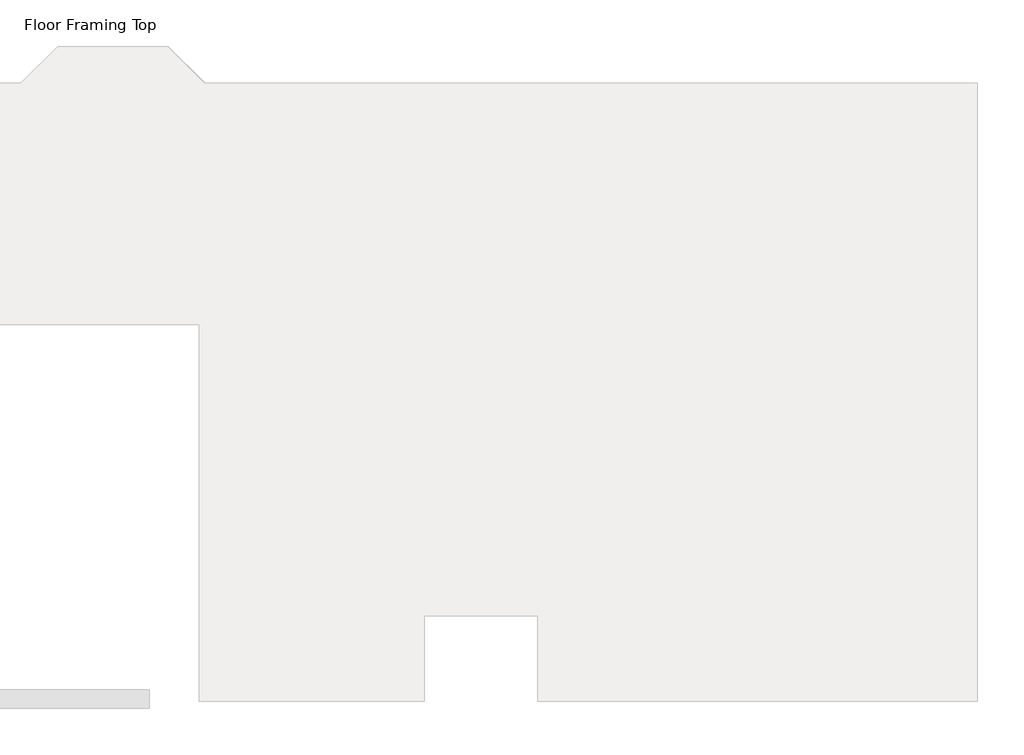
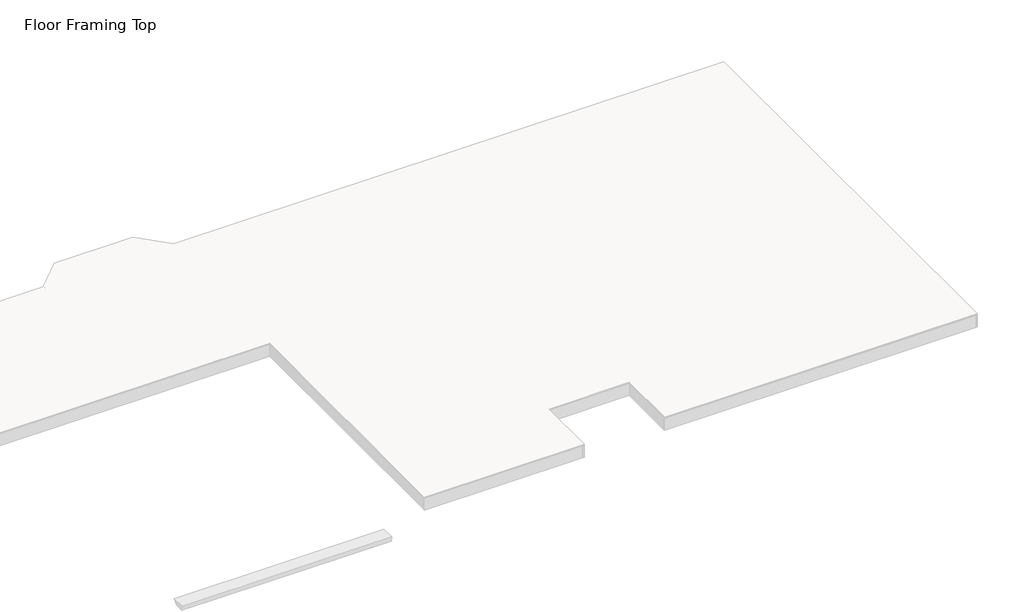
# One storey, part 2 of 4: 23 beams.
"""IFC4 building model written with IfcOpenShell, lengths in millimetres."""

import ifcopenshell
import ifcopenshell.guid

model = None  # the IFC model being written
_history = None  # IfcOwnerHistory: only IFC2X3 demands one
_inside = {}  # id of a spatial element -> (the spatial element, [elements in it])
_under = {}  # id of a project, library or spatial element -> (it, [spatial elements below it])
_declared = {}  # id of a project -> (the project, [libraries it declares])
_typed = {}  # id of a type object -> (the type object, [elements of that type])
_made_of = {}  # id of a material, layer set ... -> (it, [elements and type objects made of it])


def new_model(schema):
    """Start an empty IFC model of exactly this schema.

    Asked for "IFC4X3", IfcOpenShell would pick the latest addendum, in which some entities
    have other attributes; the version numbers below select the first issue.
    IFC2X3 requires an IfcOwnerHistory on every rooted entity: one is made here for all.
    """
    global model, _history
    if schema == "IFC4X3":
        model = ifcopenshell.file(schema_version=(4, 3, 0, 0))
    else:
        model = ifcopenshell.file(schema=schema)
    _inside.clear()
    _under.clear()
    _declared.clear()
    _typed.clear()
    _made_of.clear()
    _history = None
    if model.schema == "IFC2X3":
        org = make("IfcOrganization", Name="unknown")
        user = make(
            "IfcPersonAndOrganization",
            ThePerson=make("IfcPerson", FamilyName="unknown"),
            TheOrganization=org,
        )
        app = make(
            "IfcApplication",
            ApplicationDeveloper=org,
            Version="unknown",
            ApplicationFullName="unknown",
            ApplicationIdentifier="unknown",
        )
        _history = make(
            "IfcOwnerHistory",
            OwningUser=user,
            OwningApplication=app,
            ChangeAction="ADDED",
            CreationDate=0,
        )
    return model


def make(cls, **values):
    """One entity of the class cls with the attributes given. An attribute that is None is left unset."""
    return model.create_entity(
        cls, **{name: value for name, value in values.items() if value is not None}
    )


def rooted(cls, **values):
    """An entity with a GlobalId (a new one), such as an element, a storey or a relation."""
    return make(cls, GlobalId=ifcopenshell.guid.new(), OwnerHistory=_history, **values)


def si_unit(unit_type, name, prefix=None):
    """IfcSIUnit, for example si_unit("LENGTHUNIT", "METRE", prefix="MILLI")."""
    return make("IfcSIUnit", UnitType=unit_type, Prefix=prefix, Name=name)


def assignment(units):
    """IfcUnitAssignment: the units of a project."""
    return None if units is None else make("IfcUnitAssignment", Units=units)


def point(xyz):
    """IfcCartesianPoint."""
    return None if xyz is None else make("IfcCartesianPoint", Coordinates=xyz)


def direction(xyz):
    """IfcDirection."""
    return None if xyz is None else make("IfcDirection", DirectionRatios=xyz)


def frame(location, z_axis=None, x_axis=None):
    """IfcAxis2Placement3D, a coordinate frame: its origin and axes. An axis left out is left unset."""
    return make(
        "IfcAxis2Placement3D",
        Location=point(location),
        Axis=direction(z_axis),
        RefDirection=direction(x_axis),
    )


def origin():
    """The frame at (0, 0, 0) with its axes left unset."""
    return frame((0.0, 0.0, 0.0))


def place(relative_to, where):
    """IfcLocalPlacement: puts the frame where relative to a parent placement (None: the world)."""
    return make(
        "IfcLocalPlacement", PlacementRelTo=relative_to, RelativePlacement=where
    )


def context(
    kind, dimensions, precision=None, world=None, true_north=None, identifier=None
):
    """IfcGeometricRepresentationContext, for example the 3D "Model" context."""
    return make(
        "IfcGeometricRepresentationContext",
        ContextIdentifier=identifier,
        ContextType=kind,
        CoordinateSpaceDimension=dimensions,
        Precision=precision,
        WorldCoordinateSystem=world,
        TrueNorth=true_north,
    )


def project(units=None, contexts=None):
    """IfcProject with its units and contexts."""
    return rooted(
        "IfcProject",
        Name="project",
        RepresentationContexts=contexts,
        UnitsInContext=assignment(units),
    )


def spatial(cls, under=None, at=None, **own):
    """A site, building, storey or space (cls), placed at a placement, below another one or the project."""
    s = rooted(cls, ObjectPlacement=at, **own)
    if under is not None:
        _under.setdefault(under.id(), (under, []))[1].append(s)
    return s


def polyline(points):
    """IfcPolyline through the points."""
    return make("IfcPolyline", Points=[point(p) for p in points])


def outline(outer, holes=None, kind="AREA"):
    """IfcArbitraryClosedProfileDef: a profile drawn as a closed curve; with holes, ...WithVoids."""
    if holes is None:
        return make("IfcArbitraryClosedProfileDef", ProfileType=kind, OuterCurve=outer)
    return make(
        "IfcArbitraryProfileDefWithVoids",
        ProfileType=kind,
        OuterCurve=outer,
        InnerCurves=holes,
    )


def extrude(swept, where, along, depth):
    """IfcExtrudedAreaSolid: the profile swept, set in the frame where, extruded along a direction by depth."""
    return make(
        "IfcExtrudedAreaSolid",
        SweptArea=swept,
        Position=where,
        ExtrudedDirection=direction(along),
        Depth=depth,
    )


def shape(context_of_items, identifier, shape_type, items):
    """IfcShapeRepresentation: the items that make up one representation, for example the "Body"."""
    return make(
        "IfcShapeRepresentation",
        ContextOfItems=context_of_items,
        RepresentationIdentifier=identifier,
        RepresentationType=shape_type,
        Items=items,
    )


def source(mapping_origin, context_of_items, identifier, shape_type, items):
    """IfcRepresentationMap: a shape defined once, which mapped items show again and again."""
    return make(
        "IfcRepresentationMap",
        MappingOrigin=mapping_origin,
        MappedRepresentation=shape(context_of_items, identifier, shape_type, items),
    )


def transform(
    local_origin,
    x_axis=None,
    y_axis=None,
    z_axis=None,
    scale=None,
    scale2=None,
    scale3=None,
    uniform=True,
):
    """IfcCartesianTransformationOperator3D, or its non-uniform kind. x_axis, y_axis, z_axis: its Axis1, 2, 3."""
    if uniform:
        return make(
            "IfcCartesianTransformationOperator3D",
            Axis1=direction(x_axis),
            Axis2=direction(y_axis),
            LocalOrigin=point(local_origin),
            Scale=scale,
            Axis3=direction(z_axis),
        )
    return make(
        "IfcCartesianTransformationOperator3DnonUniform",
        Axis1=direction(x_axis),
        Axis2=direction(y_axis),
        LocalOrigin=point(local_origin),
        Scale=scale,
        Axis3=direction(z_axis),
        Scale2=scale2,
        Scale3=scale3,
    )


def mapped(mapping_source, mapping_target):
    """IfcMappedItem: shows the shape of a source again, moved by a transform."""
    return make(
        "IfcMappedItem", MappingSource=mapping_source, MappingTarget=mapping_target
    )


def made_of(thing, what):
    """Note that an element or type object is made of a material, layer set ...; save() writes the relation."""
    if what is not None:
        _made_of.setdefault(what.id(), (what, []))[1].append(thing)
    return thing


def element(
    cls,
    number,
    at=None,
    inside=None,
    cuts=None,
    type_object=None,
    material=None,
    context=None,
    identifier="Body",
    shape_type=None,
    held_by="IfcProductDefinitionShape",
    body=None,
    shapes=None,
    **own,
):
    """One element of the class cls, such as IfcWall. Its Tag is "e" and its number.

    at: its placement. inside: the storey or other place that contains it. cuts: it is an
    opening in that element (IfcRelVoidsElement). A single representation is given by context,
    identifier, shape_type and body (its items); several are given by shapes. held_by: the class
    of the entity that holds the representations. save() writes the other relations.
    """
    e = rooted(cls, Tag="e%d" % number, ObjectPlacement=at, **own)
    if body is not None:
        shapes = [shape(context, identifier, shape_type, body)]
    if shapes is not None:
        e.Representation = make(held_by, Representations=shapes)
    if inside is not None:
        _inside.setdefault(inside.id(), (inside, []))[1].append(e)
    if cuts is not None:
        rooted(
            "IfcRelVoidsElement", RelatingBuildingElement=cuts, RelatedOpeningElement=e
        )
    if type_object is not None:
        _typed.setdefault(type_object.id(), (type_object, []))[1].append(e)
    return made_of(e, material)


def aggregate(whole, parts):
    """IfcRelAggregates: a whole, such as a stair, and the parts it consists of."""
    return rooted("IfcRelAggregates", RelatingObject=whole, RelatedObjects=parts)


def save(model, path):
    """Write the relations noted so far, then the file.

    IfcRelAggregates (storeys below a building ...), IfcRelContainedInSpatialStructure (elements
    in a storey), IfcRelDefinesByType, IfcRelAssociatesMaterial and IfcRelDeclares: one each for
    every whole, place, type object, material and project.
    """
    for whole, parts in _under.values():
        aggregate(whole, parts)
    for where, things in _inside.values():
        rooted(
            "IfcRelContainedInSpatialStructure",
            RelatedElements=things,
            RelatingStructure=where,
        )
    for kind, things in _typed.values():
        rooted("IfcRelDefinesByType", RelatedObjects=things, RelatingType=kind)
    for what, things in _made_of.values():
        rooted("IfcRelAssociatesMaterial", RelatedObjects=things, RelatingMaterial=what)
    for by, libraries in _declared.values():
        rooted("IfcRelDeclares", RelatingContext=by, RelatedDefinitions=libraries)
    model.write(path)


def plywood_web_joist_11_7_8_tji_150_6827b9fe(model_context):
    return source(origin(), model_context, "Body", "SweptSolid", [
        extrude(outline(polyline([(-19.05, 150.8125), (19.05, 150.8125), (19.05, 112.7125), (4.7625, 112.7125), (4.7625, 119.0625), (-4.7625, 119.0625), (-4.7625, 112.7125), (-19.05, 112.7125), (-19.05, 150.8125)])), frame((-6407.15, 0.0, 0.0), z_axis=(1.0, 0.0, 0.0), x_axis=(0.0, 1.0, 0.0)), (0.0, 0.0, 1.0), 12812.7125),
        extrude(outline(polyline([(19.05, -112.7125), (19.05, -150.8125), (-19.05, -150.8125), (-19.05, -112.7125), (-4.7625, -112.7125), (-4.7625, -118.3285374), (4.7625, -118.3285374), (4.7625, -112.7125), (19.05, -112.7125)])), frame((-6407.15, 0.0, 0.0), z_axis=(1.0, 0.0, 0.0), x_axis=(0.0, 1.0, 0.0)), (0.0, 0.0, 1.0), 12812.7125),
        extrude(outline(polyline([(6405.5625, 4.7625), (6405.5625, -4.7625), (-6407.15, -4.7625), (-6407.15, 4.7625), (6405.5625, 4.7625)])), frame((0.0, 0.0, -118.3285374), z_axis=(0.0, 0.0, 1.0), x_axis=(1.0, 0.0, 0.0)), (0.0, 0.0, 1.0), 237.3910374),
    ])


model = new_model("IFC4")

# Units and contexts
model_context = context("Model", 3, world=origin())
ifc_project = project(units=[si_unit("LENGTHUNIT", "METRE", prefix="MILLI")], contexts=[model_context])

# Site, building, storey
site = spatial("IfcSite", under=ifc_project)
building = spatial("IfcBuilding", under=site)
storey = spatial("IfcBuildingStorey", under=building, Name="Floor Framing Top", Elevation=0.0)

# Beams
placement = place(None, origin())
element("IfcBeam", 1, ObjectType="Plywood Web Joist : 11 7/8 TJI 150", at=placement, inside=storey, context=model_context, shape_type="SweptSolid", body=[
    extrude(outline(polyline([(7976.7472749, -5717.8040947), (7967.2222749, -5717.8040947), (7967.2222749, 4456.4834053), (7976.7472749, 4456.4834053), (7976.7472749, -5717.8040947)])), frame((0.0, 0.0, -269.1410374), z_axis=(0.0, 0.0, 1.0), x_axis=(1.0, 0.0, 0.0)), (0.0, 0.0, 1.0), 237.3910374),
    extrude(outline(polyline([(7967.2222749, -663.2040947), (7967.2222749, 4456.4834053), (7976.7472749, 4456.4834053), (7976.7472749, -663.2040947), (7967.2222749, -663.2040947)])), frame((0.0, 0.0, -269.1410374), z_axis=(0.0, 0.0, 1.0), x_axis=(1.0, 0.0, 0.0)), (0.0, 0.0, 1.0), 237.3910374),
    extrude(outline(polyline([(0.0, 7952.9347749), (-38.1, 7952.9347749), (-38.1, 7967.2222749), (-31.75, 7967.2222749), (-31.75, 7976.7472749), (-38.1, 7976.7472749), (-38.1, 7991.0347749), (0.0, 7991.0347749), (0.0, 7952.9347749)])), frame((0.0, -5717.8040947, 0.0), z_axis=(0.0, 1.0, 0.0), x_axis=(0.0, 0.0, 1.0)), (0.0, 0.0, 1.0), 10174.2875),
    extrude(outline(polyline([(-263.525, 7991.0347749), (-263.525, 7976.7472749), (-269.1410374, 7976.7472749), (-269.1410374, 7967.2222749), (-263.525, 7967.2222749), (-263.525, 7952.9347749), (-301.625, 7952.9347749), (-301.625, 7991.0347749), (-263.525, 7991.0347749)])), frame((0.0, -5717.8040947, 0.0), z_axis=(0.0, 1.0, 0.0), x_axis=(0.0, 0.0, 1.0)), (0.0, 0.0, 1.0), 10174.2875),
    extrude(outline(polyline([(0.0, 7952.9347749), (-38.1, 7952.9347749), (-38.1, 7967.2222749), (-31.75, 7967.2222749), (-31.75, 7976.7472749), (-38.1, 7976.7472749), (-38.1, 7991.0347749), (0.0, 7991.0347749), (0.0, 7952.9347749)])), frame((0.0, -663.2040947, 0.0), z_axis=(0.0, 1.0, 0.0), x_axis=(0.0, 0.0, 1.0)), (0.0, 0.0, 1.0), 5119.6875),
    extrude(outline(polyline([(-263.525, 7991.0347749), (-263.525, 7976.7472749), (-269.1410374, 7976.7472749), (-269.1410374, 7967.2222749), (-263.525, 7967.2222749), (-263.525, 7952.9347749), (-301.625, 7952.9347749), (-301.625, 7991.0347749), (-263.525, 7991.0347749)])), frame((0.0, -663.2040947, 0.0), z_axis=(0.0, 1.0, 0.0), x_axis=(0.0, 0.0, 1.0)), (0.0, 0.0, 1.0), 5119.6875),
])
element("IfcBeam", 2, ObjectType="Plywood Web Joist : 11 7/8 TJI 150", at=placement, inside=storey, context=model_context, shape_type="SweptSolid", body=[
    extrude(outline(polyline([(7570.3472749, -5717.8040947), (7560.8222749, -5717.8040947), (7560.8222749, 4456.4834053), (7570.3472749, 4456.4834053), (7570.3472749, -5717.8040947)])), frame((0.0, 0.0, -269.1410374), z_axis=(0.0, 0.0, 1.0), x_axis=(1.0, 0.0, 0.0)), (0.0, 0.0, 1.0), 237.3910374),
    extrude(outline(polyline([(7560.8222749, -663.2040947), (7560.8222749, 4456.4834053), (7570.3472749, 4456.4834053), (7570.3472749, -663.2040947), (7560.8222749, -663.2040947)])), frame((0.0, 0.0, -269.1410374), z_axis=(0.0, 0.0, 1.0), x_axis=(1.0, 0.0, 0.0)), (0.0, 0.0, 1.0), 237.3910374),
    extrude(outline(polyline([(0.0, 7546.5347749), (-38.1, 7546.5347749), (-38.1, 7560.8222749), (-31.75, 7560.8222749), (-31.75, 7570.3472749), (-38.1, 7570.3472749), (-38.1, 7584.6347749), (0.0, 7584.6347749), (0.0, 7546.5347749)])), frame((0.0, -5717.8040947, 0.0), z_axis=(0.0, 1.0, 0.0), x_axis=(0.0, 0.0, 1.0)), (0.0, 0.0, 1.0), 10174.2875),
    extrude(outline(polyline([(-263.525, 7584.6347749), (-263.525, 7570.3472749), (-269.1410374, 7570.3472749), (-269.1410374, 7560.8222749), (-263.525, 7560.8222749), (-263.525, 7546.5347749), (-301.625, 7546.5347749), (-301.625, 7584.6347749), (-263.525, 7584.6347749)])), frame((0.0, -5717.8040947, 0.0), z_axis=(0.0, 1.0, 0.0), x_axis=(0.0, 0.0, 1.0)), (0.0, 0.0, 1.0), 10174.2875),
    extrude(outline(polyline([(0.0, 7546.5347749), (-38.1, 7546.5347749), (-38.1, 7560.8222749), (-31.75, 7560.8222749), (-31.75, 7570.3472749), (-38.1, 7570.3472749), (-38.1, 7584.6347749), (0.0, 7584.6347749), (0.0, 7546.5347749)])), frame((0.0, -663.2040947, 0.0), z_axis=(0.0, 1.0, 0.0), x_axis=(0.0, 0.0, 1.0)), (0.0, 0.0, 1.0), 5119.6875),
    extrude(outline(polyline([(-263.525, 7584.6347749), (-263.525, 7570.3472749), (-269.1410374, 7570.3472749), (-269.1410374, 7560.8222749), (-263.525, 7560.8222749), (-263.525, 7546.5347749), (-301.625, 7546.5347749), (-301.625, 7584.6347749), (-263.525, 7584.6347749)])), frame((0.0, -663.2040947, 0.0), z_axis=(0.0, 1.0, 0.0), x_axis=(0.0, 0.0, 1.0)), (0.0, 0.0, 1.0), 5119.6875),
])
element("IfcBeam", 3, ObjectType="Plywood Web Joist : 11 7/8 TJI 150", at=placement, inside=storey, context=model_context, shape_type="SweptSolid", body=[
    extrude(outline(polyline([(7163.9472749, -5717.8040947), (7154.4222749, -5717.8040947), (7154.4222749, 4456.4834053), (7163.9472749, 4456.4834053), (7163.9472749, -5717.8040947)])), frame((0.0, 0.0, -269.1410374), z_axis=(0.0, 0.0, 1.0), x_axis=(1.0, 0.0, 0.0)), (0.0, 0.0, 1.0), 237.3910374),
    extrude(outline(polyline([(7154.4222749, -663.2040947), (7154.4222749, 4456.4834053), (7163.9472749, 4456.4834053), (7163.9472749, -663.2040947), (7154.4222749, -663.2040947)])), frame((0.0, 0.0, -269.1410374), z_axis=(0.0, 0.0, 1.0), x_axis=(1.0, 0.0, 0.0)), (0.0, 0.0, 1.0), 237.3910374),
    extrude(outline(polyline([(0.0, 7140.1347749), (-38.1, 7140.1347749), (-38.1, 7154.4222749), (-31.75, 7154.4222749), (-31.75, 7163.9472749), (-38.1, 7163.9472749), (-38.1, 7178.2347749), (0.0, 7178.2347749), (0.0, 7140.1347749)])), frame((0.0, -5717.8040947, 0.0), z_axis=(0.0, 1.0, 0.0), x_axis=(0.0, 0.0, 1.0)), (0.0, 0.0, 1.0), 10174.2875),
    extrude(outline(polyline([(-263.525, 7178.2347749), (-263.525, 7163.9472749), (-269.1410374, 7163.9472749), (-269.1410374, 7154.4222749), (-263.525, 7154.4222749), (-263.525, 7140.1347749), (-301.625, 7140.1347749), (-301.625, 7178.2347749), (-263.525, 7178.2347749)])), frame((0.0, -5717.8040947, 0.0), z_axis=(0.0, 1.0, 0.0), x_axis=(0.0, 0.0, 1.0)), (0.0, 0.0, 1.0), 10174.2875),
    extrude(outline(polyline([(0.0, 7140.1347749), (-38.1, 7140.1347749), (-38.1, 7154.4222749), (-31.75, 7154.4222749), (-31.75, 7163.9472749), (-38.1, 7163.9472749), (-38.1, 7178.2347749), (0.0, 7178.2347749), (0.0, 7140.1347749)])), frame((0.0, -663.2040947, 0.0), z_axis=(0.0, 1.0, 0.0), x_axis=(0.0, 0.0, 1.0)), (0.0, 0.0, 1.0), 5119.6875),
    extrude(outline(polyline([(-263.525, 7178.2347749), (-263.525, 7163.9472749), (-269.1410374, 7163.9472749), (-269.1410374, 7154.4222749), (-263.525, 7154.4222749), (-263.525, 7140.1347749), (-301.625, 7140.1347749), (-301.625, 7178.2347749), (-263.525, 7178.2347749)])), frame((0.0, -663.2040947, 0.0), z_axis=(0.0, 1.0, 0.0), x_axis=(0.0, 0.0, 1.0)), (0.0, 0.0, 1.0), 5119.6875),
])
element("IfcBeam", 4, ObjectType="Plywood Web Joist : 11 7/8 TJI 150", at=placement, inside=storey, context=model_context, shape_type="SweptSolid", body=[
    extrude(outline(polyline([(6757.5472749, -5717.8040947), (6748.0222749, -5717.8040947), (6748.0222749, 4456.4834053), (6757.5472749, 4456.4834053), (6757.5472749, -5717.8040947)])), frame((0.0, 0.0, -269.1410374), z_axis=(0.0, 0.0, 1.0), x_axis=(1.0, 0.0, 0.0)), (0.0, 0.0, 1.0), 237.3910374),
    extrude(outline(polyline([(6748.0222749, -663.2040947), (6748.0222749, 4456.4834053), (6757.5472749, 4456.4834053), (6757.5472749, -663.2040947), (6748.0222749, -663.2040947)])), frame((0.0, 0.0, -269.1410374), z_axis=(0.0, 0.0, 1.0), x_axis=(1.0, 0.0, 0.0)), (0.0, 0.0, 1.0), 237.3910374),
    extrude(outline(polyline([(0.0, 6733.7347749), (-38.1, 6733.7347749), (-38.1, 6748.0222749), (-31.75, 6748.0222749), (-31.75, 6757.5472749), (-38.1, 6757.5472749), (-38.1, 6771.8347749), (0.0, 6771.8347749), (0.0, 6733.7347749)])), frame((0.0, -5717.8040947, 0.0), z_axis=(0.0, 1.0, 0.0), x_axis=(0.0, 0.0, 1.0)), (0.0, 0.0, 1.0), 10174.2875),
    extrude(outline(polyline([(-263.525, 6771.8347749), (-263.525, 6757.5472749), (-269.1410374, 6757.5472749), (-269.1410374, 6748.0222749), (-263.525, 6748.0222749), (-263.525, 6733.7347749), (-301.625, 6733.7347749), (-301.625, 6771.8347749), (-263.525, 6771.8347749)])), frame((0.0, -5717.8040947, 0.0), z_axis=(0.0, 1.0, 0.0), x_axis=(0.0, 0.0, 1.0)), (0.0, 0.0, 1.0), 10174.2875),
    extrude(outline(polyline([(0.0, 6733.7347749), (-38.1, 6733.7347749), (-38.1, 6748.0222749), (-31.75, 6748.0222749), (-31.75, 6757.5472749), (-38.1, 6757.5472749), (-38.1, 6771.8347749), (0.0, 6771.8347749), (0.0, 6733.7347749)])), frame((0.0, -663.2040947, 0.0), z_axis=(0.0, 1.0, 0.0), x_axis=(0.0, 0.0, 1.0)), (0.0, 0.0, 1.0), 5119.6875),
    extrude(outline(polyline([(-263.525, 6771.8347749), (-263.525, 6757.5472749), (-269.1410374, 6757.5472749), (-269.1410374, 6748.0222749), (-263.525, 6748.0222749), (-263.525, 6733.7347749), (-301.625, 6733.7347749), (-301.625, 6771.8347749), (-263.525, 6771.8347749)])), frame((0.0, -663.2040947, 0.0), z_axis=(0.0, 1.0, 0.0), x_axis=(0.0, 0.0, 1.0)), (0.0, 0.0, 1.0), 5119.6875),
])
element("IfcBeam", 5, ObjectType="Plywood Web Joist : 11 7/8 TJI 150", at=placement, inside=storey, context=model_context, shape_type="SweptSolid", body=[
    extrude(outline(polyline([(6351.1472749, -5717.8040947), (6341.6222749, -5717.8040947), (6341.6222749, 4456.4834053), (6351.1472749, 4456.4834053), (6351.1472749, -5717.8040947)])), frame((0.0, 0.0, -269.1410374), z_axis=(0.0, 0.0, 1.0), x_axis=(1.0, 0.0, 0.0)), (0.0, 0.0, 1.0), 237.3910374),
    extrude(outline(polyline([(6341.6222749, -663.2040947), (6341.6222749, 4456.4834053), (6351.1472749, 4456.4834053), (6351.1472749, -663.2040947), (6341.6222749, -663.2040947)])), frame((0.0, 0.0, -269.1410374), z_axis=(0.0, 0.0, 1.0), x_axis=(1.0, 0.0, 0.0)), (0.0, 0.0, 1.0), 237.3910374),
    extrude(outline(polyline([(0.0, 6327.3347749), (-38.1, 6327.3347749), (-38.1, 6341.6222749), (-31.75, 6341.6222749), (-31.75, 6351.1472749), (-38.1, 6351.1472749), (-38.1, 6365.4347749), (0.0, 6365.4347749), (0.0, 6327.3347749)])), frame((0.0, -5717.8040947, 0.0), z_axis=(0.0, 1.0, 0.0), x_axis=(0.0, 0.0, 1.0)), (0.0, 0.0, 1.0), 10174.2875),
    extrude(outline(polyline([(-263.525, 6365.4347749), (-263.525, 6351.1472749), (-269.1410374, 6351.1472749), (-269.1410374, 6341.6222749), (-263.525, 6341.6222749), (-263.525, 6327.3347749), (-301.625, 6327.3347749), (-301.625, 6365.4347749), (-263.525, 6365.4347749)])), frame((0.0, -5717.8040947, 0.0), z_axis=(0.0, 1.0, 0.0), x_axis=(0.0, 0.0, 1.0)), (0.0, 0.0, 1.0), 10174.2875),
    extrude(outline(polyline([(0.0, 6327.3347749), (-38.1, 6327.3347749), (-38.1, 6341.6222749), (-31.75, 6341.6222749), (-31.75, 6351.1472749), (-38.1, 6351.1472749), (-38.1, 6365.4347749), (0.0, 6365.4347749), (0.0, 6327.3347749)])), frame((0.0, -663.2040947, 0.0), z_axis=(0.0, 1.0, 0.0), x_axis=(0.0, 0.0, 1.0)), (0.0, 0.0, 1.0), 5119.6875),
    extrude(outline(polyline([(-263.525, 6365.4347749), (-263.525, 6351.1472749), (-269.1410374, 6351.1472749), (-269.1410374, 6341.6222749), (-263.525, 6341.6222749), (-263.525, 6327.3347749), (-301.625, 6327.3347749), (-301.625, 6365.4347749), (-263.525, 6365.4347749)])), frame((0.0, -663.2040947, 0.0), z_axis=(0.0, 1.0, 0.0), x_axis=(0.0, 0.0, 1.0)), (0.0, 0.0, 1.0), 5119.6875),
])
element("IfcBeam", 6, ObjectType="Plywood Web Joist : 11 7/8 TJI 150", at=placement, inside=storey, context=model_context, shape_type="SweptSolid", body=[
    extrude(outline(polyline([(3099.9472749, -5717.8040947), (3090.4222749, -5717.8040947), (3090.4222749, 4456.4834053), (3099.9472749, 4456.4834053), (3099.9472749, -5717.8040947)])), frame((0.0, 0.0, -269.1410374), z_axis=(0.0, 0.0, 1.0), x_axis=(1.0, 0.0, 0.0)), (0.0, 0.0, 1.0), 237.3910374),
    extrude(outline(polyline([(3090.4222749, -663.2040947), (3090.4222749, 4456.4834053), (3099.9472749, 4456.4834053), (3099.9472749, -663.2040947), (3090.4222749, -663.2040947)])), frame((0.0, 0.0, -269.1410374), z_axis=(0.0, 0.0, 1.0), x_axis=(1.0, 0.0, 0.0)), (0.0, 0.0, 1.0), 237.3910374),
    extrude(outline(polyline([(0.0, 3076.1347749), (-38.1, 3076.1347749), (-38.1, 3090.4222749), (-31.75, 3090.4222749), (-31.75, 3099.9472749), (-38.1, 3099.9472749), (-38.1, 3114.2347749), (0.0, 3114.2347749), (0.0, 3076.1347749)])), frame((0.0, -5717.8040947, 0.0), z_axis=(0.0, 1.0, 0.0), x_axis=(0.0, 0.0, 1.0)), (0.0, 0.0, 1.0), 10174.2875),
    extrude(outline(polyline([(-263.525, 3114.2347749), (-263.525, 3099.9472749), (-269.1410374, 3099.9472749), (-269.1410374, 3090.4222749), (-263.525, 3090.4222749), (-263.525, 3076.1347749), (-301.625, 3076.1347749), (-301.625, 3114.2347749), (-263.525, 3114.2347749)])), frame((0.0, -5717.8040947, 0.0), z_axis=(0.0, 1.0, 0.0), x_axis=(0.0, 0.0, 1.0)), (0.0, 0.0, 1.0), 10174.2875),
    extrude(outline(polyline([(0.0, 3076.1347749), (-38.1, 3076.1347749), (-38.1, 3090.4222749), (-31.75, 3090.4222749), (-31.75, 3099.9472749), (-38.1, 3099.9472749), (-38.1, 3114.2347749), (0.0, 3114.2347749), (0.0, 3076.1347749)])), frame((0.0, -663.2040947, 0.0), z_axis=(0.0, 1.0, 0.0), x_axis=(0.0, 0.0, 1.0)), (0.0, 0.0, 1.0), 5119.6875),
    extrude(outline(polyline([(-263.525, 3114.2347749), (-263.525, 3099.9472749), (-269.1410374, 3099.9472749), (-269.1410374, 3090.4222749), (-263.525, 3090.4222749), (-263.525, 3076.1347749), (-301.625, 3076.1347749), (-301.625, 3114.2347749), (-263.525, 3114.2347749)])), frame((0.0, -663.2040947, 0.0), z_axis=(0.0, 1.0, 0.0), x_axis=(0.0, 0.0, 1.0)), (0.0, 0.0, 1.0), 5119.6875),
])
element("IfcBeam", 7, ObjectType="Plywood Web Joist : 11 7/8 TJI 150", at=placement, inside=storey, context=model_context, shape_type="SweptSolid", body=[
    extrude(outline(polyline([(4319.1472749, -701.3040947), (4319.1472749, -4295.4040947), (4309.6222749, -4295.4040947), (4309.6222749, -701.3040947), (4319.1472749, -701.3040947)])), frame((0.0, 0.0, -269.1410374), z_axis=(0.0, 0.0, 1.0), x_axis=(1.0, 0.0, 0.0)), (0.0, 0.0, 1.0), 237.3910374),
    extrude(outline(polyline([(0.0, 4295.3347749), (-38.1, 4295.3347749), (-38.1, 4309.6222749), (-31.75, 4309.6222749), (-31.75, 4319.1472749), (-38.1, 4319.1472749), (-38.1, 4333.4347749), (0.0, 4333.4347749), (0.0, 4295.3347749)])), frame((0.0, -4295.4040947, 0.0), z_axis=(0.0, 1.0, 0.0), x_axis=(0.0, 0.0, 1.0)), (0.0, 0.0, 1.0), 3594.1),
    extrude(outline(polyline([(-263.525, 4333.4347749), (-263.525, 4319.1472749), (-269.1410374, 4319.1472749), (-269.1410374, 4309.6222749), (-263.525, 4309.6222749), (-263.525, 4295.3347749), (-301.625, 4295.3347749), (-301.625, 4333.4347749), (-263.525, 4333.4347749)])), frame((0.0, -4295.4040947, 0.0), z_axis=(0.0, 1.0, 0.0), x_axis=(0.0, 0.0, 1.0)), (0.0, 0.0, 1.0), 3594.1),
])
element("IfcBeam", 8, ObjectType="Plywood Web Joist : 11 7/8 TJI 150", at=placement, inside=storey, context=model_context, shape_type="SweptSolid", body=[
    extrude(outline(polyline([(4725.5472749, -701.3040947), (4725.5472749, -4295.4040947), (4716.0222749, -4295.4040947), (4716.0222749, -701.3040947), (4725.5472749, -701.3040947)])), frame((0.0, 0.0, -269.1410374), z_axis=(0.0, 0.0, 1.0), x_axis=(1.0, 0.0, 0.0)), (0.0, 0.0, 1.0), 237.3910374),
    extrude(outline(polyline([(0.0, 4701.7347749), (-38.1, 4701.7347749), (-38.1, 4716.0222749), (-31.75, 4716.0222749), (-31.75, 4725.5472749), (-38.1, 4725.5472749), (-38.1, 4739.8347749), (0.0, 4739.8347749), (0.0, 4701.7347749)])), frame((0.0, -4295.4040947, 0.0), z_axis=(0.0, 1.0, 0.0), x_axis=(0.0, 0.0, 1.0)), (0.0, 0.0, 1.0), 3594.1),
    extrude(outline(polyline([(-263.525, 4739.8347749), (-263.525, 4725.5472749), (-269.1410374, 4725.5472749), (-269.1410374, 4716.0222749), (-263.525, 4716.0222749), (-263.525, 4701.7347749), (-301.625, 4701.7347749), (-301.625, 4739.8347749), (-263.525, 4739.8347749)])), frame((0.0, -4295.4040947, 0.0), z_axis=(0.0, 1.0, 0.0), x_axis=(0.0, 0.0, 1.0)), (0.0, 0.0, 1.0), 3594.1),
])
element("IfcBeam", 9, ObjectType="Plywood Web Joist : 11 7/8 TJI 150", at=placement, inside=storey, context=model_context, shape_type="SweptSolid", body=[
    extrude(outline(polyline([(5131.9472749, -701.3040947), (5131.9472749, -4295.4040947), (5122.4222749, -4295.4040947), (5122.4222749, -701.3040947), (5131.9472749, -701.3040947)])), frame((0.0, 0.0, -269.1410374), z_axis=(0.0, 0.0, 1.0), x_axis=(1.0, 0.0, 0.0)), (0.0, 0.0, 1.0), 237.3910374),
    extrude(outline(polyline([(0.0, 5108.1347749), (-38.1, 5108.1347749), (-38.1, 5122.4222749), (-31.75, 5122.4222749), (-31.75, 5131.9472749), (-38.1, 5131.9472749), (-38.1, 5146.2347749), (0.0, 5146.2347749), (0.0, 5108.1347749)])), frame((0.0, -4295.4040947, 0.0), z_axis=(0.0, 1.0, 0.0), x_axis=(0.0, 0.0, 1.0)), (0.0, 0.0, 1.0), 3594.1),
    extrude(outline(polyline([(-263.525, 5146.2347749), (-263.525, 5131.9472749), (-269.1410374, 5131.9472749), (-269.1410374, 5122.4222749), (-263.525, 5122.4222749), (-263.525, 5108.1347749), (-301.625, 5108.1347749), (-301.625, 5146.2347749), (-263.525, 5146.2347749)])), frame((0.0, -4295.4040947, 0.0), z_axis=(0.0, 1.0, 0.0), x_axis=(0.0, 0.0, 1.0)), (0.0, 0.0, 1.0), 3594.1),
])
element("IfcBeam", 10, ObjectType="Plywood Web Joist : 11 7/8 TJI 150", at=placement, inside=storey, context=model_context, shape_type="SweptSolid", body=[
    extrude(outline(polyline([(5538.3472749, -701.3040947), (5538.3472749, -4295.4040947), (5528.8222749, -4295.4040947), (5528.8222749, -701.3040947), (5538.3472749, -701.3040947)])), frame((0.0, 0.0, -269.1410374), z_axis=(0.0, 0.0, 1.0), x_axis=(1.0, 0.0, 0.0)), (0.0, 0.0, 1.0), 237.3910374),
    extrude(outline(polyline([(0.0, 5514.5347749), (-38.1, 5514.5347749), (-38.1, 5528.8222749), (-31.75, 5528.8222749), (-31.75, 5538.3472749), (-38.1, 5538.3472749), (-38.1, 5552.6347749), (0.0, 5552.6347749), (0.0, 5514.5347749)])), frame((0.0, -4295.4040947, 0.0), z_axis=(0.0, 1.0, 0.0), x_axis=(0.0, 0.0, 1.0)), (0.0, 0.0, 1.0), 3594.1),
    extrude(outline(polyline([(-263.525, 5552.6347749), (-263.525, 5538.3472749), (-269.1410374, 5538.3472749), (-269.1410374, 5528.8222749), (-263.525, 5528.8222749), (-263.525, 5514.5347749), (-301.625, 5514.5347749), (-301.625, 5552.6347749), (-263.525, 5552.6347749)])), frame((0.0, -4295.4040947, 0.0), z_axis=(0.0, 1.0, 0.0), x_axis=(0.0, 0.0, 1.0)), (0.0, 0.0, 1.0), 3594.1),
])
element("IfcBeam", 11, ObjectType="Plywood Web Joist : 11 7/8 TJI 150", at=placement, inside=storey, context=model_context, shape_type="SweptSolid", body=[
    extrude(outline(polyline([(5944.7472749, -701.3040947), (5944.7472749, -4295.4040947), (5935.2222749, -4295.4040947), (5935.2222749, -701.3040947), (5944.7472749, -701.3040947)])), frame((0.0, 0.0, -269.1410374), z_axis=(0.0, 0.0, 1.0), x_axis=(1.0, 0.0, 0.0)), (0.0, 0.0, 1.0), 237.3910374),
    extrude(outline(polyline([(0.0, 5920.9347749), (-38.1, 5920.9347749), (-38.1, 5935.2222749), (-31.75, 5935.2222749), (-31.75, 5944.7472749), (-38.1, 5944.7472749), (-38.1, 5959.0347749), (0.0, 5959.0347749), (0.0, 5920.9347749)])), frame((0.0, -4295.4040947, 0.0), z_axis=(0.0, 1.0, 0.0), x_axis=(0.0, 0.0, 1.0)), (0.0, 0.0, 1.0), 3594.1),
    extrude(outline(polyline([(-263.525, 5959.0347749), (-263.525, 5944.7472749), (-269.1410374, 5944.7472749), (-269.1410374, 5935.2222749), (-263.525, 5935.2222749), (-263.525, 5920.9347749), (-301.625, 5920.9347749), (-301.625, 5959.0347749), (-263.525, 5959.0347749)])), frame((0.0, -4295.4040947, 0.0), z_axis=(0.0, 1.0, 0.0), x_axis=(0.0, 0.0, 1.0)), (0.0, 0.0, 1.0), 3594.1),
])
element("IfcBeam", 12, ObjectType="Plywood Web Joist : 11 7/8 TJI 150", at=placement, inside=storey, context=model_context, shape_type="SweptSolid", body=[
    extrude(outline(polyline([(6351.1472749, -701.3040947), (6351.1472749, -5717.8040947), (6341.6222749, -5717.8040947), (6341.6222749, -701.3040947), (6351.1472749, -701.3040947)])), frame((0.0, 0.0, -269.1410374), z_axis=(0.0, 0.0, 1.0), x_axis=(1.0, 0.0, 0.0)), (0.0, 0.0, 1.0), 237.3910374),
    extrude(outline(polyline([(0.0, 6327.3347749), (-38.1, 6327.3347749), (-38.1, 6341.6222749), (-31.75, 6341.6222749), (-31.75, 6351.1472749), (-38.1, 6351.1472749), (-38.1, 6365.4347749), (0.0, 6365.4347749), (0.0, 6327.3347749)])), frame((0.0, -5717.8040947, 0.0), z_axis=(0.0, 1.0, 0.0), x_axis=(0.0, 0.0, 1.0)), (0.0, 0.0, 1.0), 5016.5),
    extrude(outline(polyline([(-263.525, 6365.4347749), (-263.525, 6351.1472749), (-269.1410374, 6351.1472749), (-269.1410374, 6341.6222749), (-263.525, 6341.6222749), (-263.525, 6327.3347749), (-301.625, 6327.3347749), (-301.625, 6365.4347749), (-263.525, 6365.4347749)])), frame((0.0, -5717.8040947, 0.0), z_axis=(0.0, 1.0, 0.0), x_axis=(0.0, 0.0, 1.0)), (0.0, 0.0, 1.0), 5016.5),
])
element("IfcBeam", 13, ObjectType="Plywood Web Joist : 11 7/8 TJI 150", at=placement, inside=storey, context=model_context, shape_type="SweptSolid", body=[
    extrude(outline(polyline([(6757.5472749, -701.3040947), (6757.5472749, -5717.8040947), (6748.0222749, -5717.8040947), (6748.0222749, -701.3040947), (6757.5472749, -701.3040947)])), frame((0.0, 0.0, -269.1410374), z_axis=(0.0, 0.0, 1.0), x_axis=(1.0, 0.0, 0.0)), (0.0, 0.0, 1.0), 237.3910374),
    extrude(outline(polyline([(0.0, 6733.7347749), (-38.1, 6733.7347749), (-38.1, 6748.0222749), (-31.75, 6748.0222749), (-31.75, 6757.5472749), (-38.1, 6757.5472749), (-38.1, 6771.8347749), (0.0, 6771.8347749), (0.0, 6733.7347749)])), frame((0.0, -5717.8040947, 0.0), z_axis=(0.0, 1.0, 0.0), x_axis=(0.0, 0.0, 1.0)), (0.0, 0.0, 1.0), 5016.5),
    extrude(outline(polyline([(-263.525, 6771.8347749), (-263.525, 6757.5472749), (-269.1410374, 6757.5472749), (-269.1410374, 6748.0222749), (-263.525, 6748.0222749), (-263.525, 6733.7347749), (-301.625, 6733.7347749), (-301.625, 6771.8347749), (-263.525, 6771.8347749)])), frame((0.0, -5717.8040947, 0.0), z_axis=(0.0, 1.0, 0.0), x_axis=(0.0, 0.0, 1.0)), (0.0, 0.0, 1.0), 5016.5),
])
element("IfcBeam", 14, ObjectType="Plywood Web Joist : 11 7/8 TJI 150", at=placement, inside=storey, context=model_context, shape_type="SweptSolid", body=[
    extrude(outline(polyline([(7163.9472749, -701.3040947), (7163.9472749, -5717.8040947), (7154.4222749, -5717.8040947), (7154.4222749, -701.3040947), (7163.9472749, -701.3040947)])), frame((0.0, 0.0, -269.1410374), z_axis=(0.0, 0.0, 1.0), x_axis=(1.0, 0.0, 0.0)), (0.0, 0.0, 1.0), 237.3910374),
    extrude(outline(polyline([(0.0, 7140.1347749), (-38.1, 7140.1347749), (-38.1, 7154.4222749), (-31.75, 7154.4222749), (-31.75, 7163.9472749), (-38.1, 7163.9472749), (-38.1, 7178.2347749), (0.0, 7178.2347749), (0.0, 7140.1347749)])), frame((0.0, -5717.8040947, 0.0), z_axis=(0.0, 1.0, 0.0), x_axis=(0.0, 0.0, 1.0)), (0.0, 0.0, 1.0), 5016.5),
    extrude(outline(polyline([(-263.525, 7178.2347749), (-263.525, 7163.9472749), (-269.1410374, 7163.9472749), (-269.1410374, 7154.4222749), (-263.525, 7154.4222749), (-263.525, 7140.1347749), (-301.625, 7140.1347749), (-301.625, 7178.2347749), (-263.525, 7178.2347749)])), frame((0.0, -5717.8040947, 0.0), z_axis=(0.0, 1.0, 0.0), x_axis=(0.0, 0.0, 1.0)), (0.0, 0.0, 1.0), 5016.5),
])
element("IfcBeam", 15, ObjectType="Plywood Web Joist : 11 7/8 TJI 150", at=placement, inside=storey, context=model_context, shape_type="SweptSolid", body=[
    extrude(outline(polyline([(7570.3472749, -701.3040947), (7570.3472749, -5717.8040947), (7560.8222749, -5717.8040947), (7560.8222749, -701.3040947), (7570.3472749, -701.3040947)])), frame((0.0, 0.0, -269.1410374), z_axis=(0.0, 0.0, 1.0), x_axis=(1.0, 0.0, 0.0)), (0.0, 0.0, 1.0), 237.3910374),
    extrude(outline(polyline([(0.0, 7546.5347749), (-38.1, 7546.5347749), (-38.1, 7560.8222749), (-31.75, 7560.8222749), (-31.75, 7570.3472749), (-38.1, 7570.3472749), (-38.1, 7584.6347749), (0.0, 7584.6347749), (0.0, 7546.5347749)])), frame((0.0, -5717.8040947, 0.0), z_axis=(0.0, 1.0, 0.0), x_axis=(0.0, 0.0, 1.0)), (0.0, 0.0, 1.0), 5016.5),
    extrude(outline(polyline([(-263.525, 7584.6347749), (-263.525, 7570.3472749), (-269.1410374, 7570.3472749), (-269.1410374, 7560.8222749), (-263.525, 7560.8222749), (-263.525, 7546.5347749), (-301.625, 7546.5347749), (-301.625, 7584.6347749), (-263.525, 7584.6347749)])), frame((0.0, -5717.8040947, 0.0), z_axis=(0.0, 1.0, 0.0), x_axis=(0.0, 0.0, 1.0)), (0.0, 0.0, 1.0), 5016.5),
])
element("IfcBeam", 16, ObjectType="Plywood Web Joist : 11 7/8 TJI 150", at=placement, inside=storey, context=model_context, shape_type="SweptSolid", body=[
    extrude(outline(polyline([(7976.7472749, -701.3040947), (7976.7472749, -5717.8040947), (7967.2222749, -5717.8040947), (7967.2222749, -701.3040947), (7976.7472749, -701.3040947)])), frame((0.0, 0.0, -269.1410374), z_axis=(0.0, 0.0, 1.0), x_axis=(1.0, 0.0, 0.0)), (0.0, 0.0, 1.0), 237.3910374),
    extrude(outline(polyline([(0.0, 7952.9347749), (-38.1, 7952.9347749), (-38.1, 7967.2222749), (-31.75, 7967.2222749), (-31.75, 7976.7472749), (-38.1, 7976.7472749), (-38.1, 7991.0347749), (0.0, 7991.0347749), (0.0, 7952.9347749)])), frame((0.0, -5717.8040947, 0.0), z_axis=(0.0, 1.0, 0.0), x_axis=(0.0, 0.0, 1.0)), (0.0, 0.0, 1.0), 5016.5),
    extrude(outline(polyline([(-263.525, 7991.0347749), (-263.525, 7976.7472749), (-269.1410374, 7976.7472749), (-269.1410374, 7967.2222749), (-263.525, 7967.2222749), (-263.525, 7952.9347749), (-301.625, 7952.9347749), (-301.625, 7991.0347749), (-263.525, 7991.0347749)])), frame((0.0, -5717.8040947, 0.0), z_axis=(0.0, 1.0, 0.0), x_axis=(0.0, 0.0, 1.0)), (0.0, 0.0, 1.0), 5016.5),
])
element("IfcBeam", 17, ObjectType="Plywood Web Joist : 11 7/8 TJI 150", at=placement, inside=storey, context=model_context, shape_type="SweptSolid", body=[
    extrude(outline(polyline([(8383.1472749, -701.3040947), (8383.1472749, -5717.8040947), (8373.6222749, -5717.8040947), (8373.6222749, -701.3040947), (8383.1472749, -701.3040947)])), frame((0.0, 0.0, -269.1410374), z_axis=(0.0, 0.0, 1.0), x_axis=(1.0, 0.0, 0.0)), (0.0, 0.0, 1.0), 237.3910374),
    extrude(outline(polyline([(0.0, 8359.3347749), (-38.1, 8359.3347749), (-38.1, 8373.6222749), (-31.75, 8373.6222749), (-31.75, 8383.1472749), (-38.1, 8383.1472749), (-38.1, 8397.4347749), (0.0, 8397.4347749), (0.0, 8359.3347749)])), frame((0.0, -5717.8040947, 0.0), z_axis=(0.0, 1.0, 0.0), x_axis=(0.0, 0.0, 1.0)), (0.0, 0.0, 1.0), 5016.5),
    extrude(outline(polyline([(-263.525, 8397.4347749), (-263.525, 8383.1472749), (-269.1410374, 8383.1472749), (-269.1410374, 8373.6222749), (-263.525, 8373.6222749), (-263.525, 8359.3347749), (-301.625, 8359.3347749), (-301.625, 8397.4347749), (-263.525, 8397.4347749)])), frame((0.0, -5717.8040947, 0.0), z_axis=(0.0, 1.0, 0.0), x_axis=(0.0, 0.0, 1.0)), (0.0, 0.0, 1.0), 5016.5),
])
element("IfcBeam", 18, ObjectType="Plywood Web Joist : 11 7/8 TJI 150", at=placement, inside=storey, context=model_context, shape_type="SweptSolid", body=[
    extrude(outline(polyline([(8789.5472749, -701.3040947), (8789.5472749, -5717.8040947), (8780.0222749, -5717.8040947), (8780.0222749, -701.3040947), (8789.5472749, -701.3040947)])), frame((0.0, 0.0, -269.1410374), z_axis=(0.0, 0.0, 1.0), x_axis=(1.0, 0.0, 0.0)), (0.0, 0.0, 1.0), 237.3910374),
    extrude(outline(polyline([(0.0, 8765.7347749), (-38.1, 8765.7347749), (-38.1, 8780.0222749), (-31.75, 8780.0222749), (-31.75, 8789.5472749), (-38.1, 8789.5472749), (-38.1, 8803.8347749), (0.0, 8803.8347749), (0.0, 8765.7347749)])), frame((0.0, -5717.8040947, 0.0), z_axis=(0.0, 1.0, 0.0), x_axis=(0.0, 0.0, 1.0)), (0.0, 0.0, 1.0), 5016.5),
    extrude(outline(polyline([(-263.525, 8803.8347749), (-263.525, 8789.5472749), (-269.1410374, 8789.5472749), (-269.1410374, 8780.0222749), (-263.525, 8780.0222749), (-263.525, 8765.7347749), (-301.625, 8765.7347749), (-301.625, 8803.8347749), (-263.525, 8803.8347749)])), frame((0.0, -5717.8040947, 0.0), z_axis=(0.0, 1.0, 0.0), x_axis=(0.0, 0.0, 1.0)), (0.0, 0.0, 1.0), 5016.5),
])
element("IfcBeam", 19, ObjectType="Plywood Web Joist : 11 7/8 TJI 150", at=placement, inside=storey, context=model_context, shape_type="SweptSolid", body=[
    extrude(outline(polyline([(9195.9472749, -701.3040947), (9195.9472749, -5717.8040947), (9186.4222749, -5717.8040947), (9186.4222749, -701.3040947), (9195.9472749, -701.3040947)])), frame((0.0, 0.0, -269.1410374), z_axis=(0.0, 0.0, 1.0), x_axis=(1.0, 0.0, 0.0)), (0.0, 0.0, 1.0), 237.3910374),
    extrude(outline(polyline([(0.0, 9172.1347749), (-38.1, 9172.1347749), (-38.1, 9186.4222749), (-31.75, 9186.4222749), (-31.75, 9195.9472749), (-38.1, 9195.9472749), (-38.1, 9210.2347749), (0.0, 9210.2347749), (0.0, 9172.1347749)])), frame((0.0, -5717.8040947, 0.0), z_axis=(0.0, 1.0, 0.0), x_axis=(0.0, 0.0, 1.0)), (0.0, 0.0, 1.0), 5016.5),
    extrude(outline(polyline([(-263.525, 9210.2347749), (-263.525, 9195.9472749), (-269.1410374, 9195.9472749), (-269.1410374, 9186.4222749), (-263.525, 9186.4222749), (-263.525, 9172.1347749), (-301.625, 9172.1347749), (-301.625, 9210.2347749), (-263.525, 9210.2347749)])), frame((0.0, -5717.8040947, 0.0), z_axis=(0.0, 1.0, 0.0), x_axis=(0.0, 0.0, 1.0)), (0.0, 0.0, 1.0), 5016.5),
])
element("IfcBeam", 20, ObjectType="Plywood Web Joist : 11 7/8 TJI 150", at=placement, inside=storey, context=model_context, shape_type="SweptSolid", body=[
    extrude(outline(polyline([(9602.3472749, -701.3040947), (9602.3472749, -5717.8040947), (9592.8222749, -5717.8040947), (9592.8222749, -701.3040947), (9602.3472749, -701.3040947)])), frame((0.0, 0.0, -269.1410374), z_axis=(0.0, 0.0, 1.0), x_axis=(1.0, 0.0, 0.0)), (0.0, 0.0, 1.0), 237.3910374),
    extrude(outline(polyline([(0.0, 9578.5347749), (-38.1, 9578.5347749), (-38.1, 9592.8222749), (-31.75, 9592.8222749), (-31.75, 9602.3472749), (-38.1, 9602.3472749), (-38.1, 9616.6347749), (0.0, 9616.6347749), (0.0, 9578.5347749)])), frame((0.0, -5717.8040947, 0.0), z_axis=(0.0, 1.0, 0.0), x_axis=(0.0, 0.0, 1.0)), (0.0, 0.0, 1.0), 5016.5),
    extrude(outline(polyline([(-263.525, 9616.6347749), (-263.525, 9602.3472749), (-269.1410374, 9602.3472749), (-269.1410374, 9592.8222749), (-263.525, 9592.8222749), (-263.525, 9578.5347749), (-301.625, 9578.5347749), (-301.625, 9616.6347749), (-263.525, 9616.6347749)])), frame((0.0, -5717.8040947, 0.0), z_axis=(0.0, 1.0, 0.0), x_axis=(0.0, 0.0, 1.0)), (0.0, 0.0, 1.0), 5016.5),
])
element("IfcBeam", 21, ObjectType="Plywood Web Joist : 11 7/8 TJI 150", at=placement, inside=storey, context=model_context, shape_type="SweptSolid", body=[
    extrude(outline(polyline([(10008.7472749, -701.3040947), (10008.7472749, -5717.8040947), (9999.2222749, -5717.8040947), (9999.2222749, -701.3040947), (10008.7472749, -701.3040947)])), frame((0.0, 0.0, -269.1410374), z_axis=(0.0, 0.0, 1.0), x_axis=(1.0, 0.0, 0.0)), (0.0, 0.0, 1.0), 237.3910374),
    extrude(outline(polyline([(0.0, 9984.9347749), (-38.1, 9984.9347749), (-38.1, 9999.2222749), (-31.75, 9999.2222749), (-31.75, 10008.7472749), (-38.1, 10008.7472749), (-38.1, 10023.0347749), (0.0, 10023.0347749), (0.0, 9984.9347749)])), frame((0.0, -5717.8040947, 0.0), z_axis=(0.0, 1.0, 0.0), x_axis=(0.0, 0.0, 1.0)), (0.0, 0.0, 1.0), 5016.5),
    extrude(outline(polyline([(-263.525, 10023.0347749), (-263.525, 10008.7472749), (-269.1410374, 10008.7472749), (-269.1410374, 9999.2222749), (-263.525, 9999.2222749), (-263.525, 9984.9347749), (-301.625, 9984.9347749), (-301.625, 10023.0347749), (-263.525, 10023.0347749)])), frame((0.0, -5717.8040947, 0.0), z_axis=(0.0, 1.0, 0.0), x_axis=(0.0, 0.0, 1.0)), (0.0, 0.0, 1.0), 5016.5),
])
element("IfcBeam", 22, ObjectType="Plywood Web Joist : 11 7/8 TJI 150", at=placement, inside=storey, context=model_context, shape_type="SweptSolid", body=[
    extrude(outline(polyline([(10415.1472749, -701.3040947), (10415.1472749, -5717.8040947), (10405.6222749, -5717.8040947), (10405.6222749, -701.3040947), (10415.1472749, -701.3040947)])), frame((0.0, 0.0, -269.1410374), z_axis=(0.0, 0.0, 1.0), x_axis=(1.0, 0.0, 0.0)), (0.0, 0.0, 1.0), 237.3910374),
    extrude(outline(polyline([(0.0, 10391.3347749), (-38.1, 10391.3347749), (-38.1, 10405.6222749), (-31.75, 10405.6222749), (-31.75, 10415.1472749), (-38.1, 10415.1472749), (-38.1, 10429.4347749), (0.0, 10429.4347749), (0.0, 10391.3347749)])), frame((0.0, -5717.8040947, 0.0), z_axis=(0.0, 1.0, 0.0), x_axis=(0.0, 0.0, 1.0)), (0.0, 0.0, 1.0), 5016.5),
    extrude(outline(polyline([(-263.525, 10429.4347749), (-263.525, 10415.1472749), (-269.1410374, 10415.1472749), (-269.1410374, 10405.6222749), (-263.525, 10405.6222749), (-263.525, 10391.3347749), (-301.625, 10391.3347749), (-301.625, 10429.4347749), (-263.525, 10429.4347749)])), frame((0.0, -5717.8040947, 0.0), z_axis=(0.0, 1.0, 0.0), x_axis=(0.0, 0.0, 1.0)), (0.0, 0.0, 1.0), 5016.5),
])
plywood_web_joist_11_7_8_tji_150_shape = plywood_web_joist_11_7_8_tji_150_6827b9fe(model_context)
element("IfcBeam", 23, ObjectType="Plywood Web Joist : 11 7/8 TJI 150", at=placement, inside=storey, context=model_context, shape_type="MappedRepresentation", body=[
    mapped(plywood_web_joist_11_7_8_tji_150_shape, transform((6805.1722749, -682.2540947, -150.8125), x_axis=(-1.0, 0.0, 0.0), y_axis=(0.0, -1.0, 0.0), z_axis=(0.0, 0.0, 1.0))),
])

save(model, "model.ifc")

# Revit data of these elements
# Type "Plywood Web Joist : 11 7/8 TJI 150"
#   Assembly Code = "B10"
#   Cost = 17.5
#   Length [instance default] = 5' - 0"
#   b = 0' - 1 1/2"
#   d = 0' - 11 7/8"
#   Structural Material [instance default] = Softwood, Lumber
# Elements 1, 2, 3, 4, 5, 6, 7, 8, 9, 10, 11, 12, 13, 14, 15, 16, 17, 18, 19, 20, 21, 22, 23 (IfcBeam, "Plywood Web Joist : 11 7/8 TJI 150")
#   Structural Material = Douglas Fir #2
#   Phase Created = New Construction
#   Materials on its faces: "Douglas Fir #2"
# Materials
#   "Softwood, Lumber": class "Wood", colour RGB 223 192 134, transparency 0, Description = "Pinus Echinata", Cost = 0
#   "Douglas Fir #2": class "Wood", colour RGB 223 192 134, transparency 0, Description = "Pinus Echinata", Cost = 0
